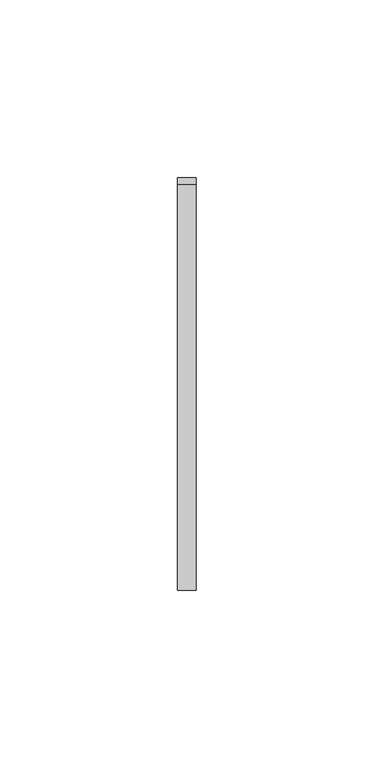
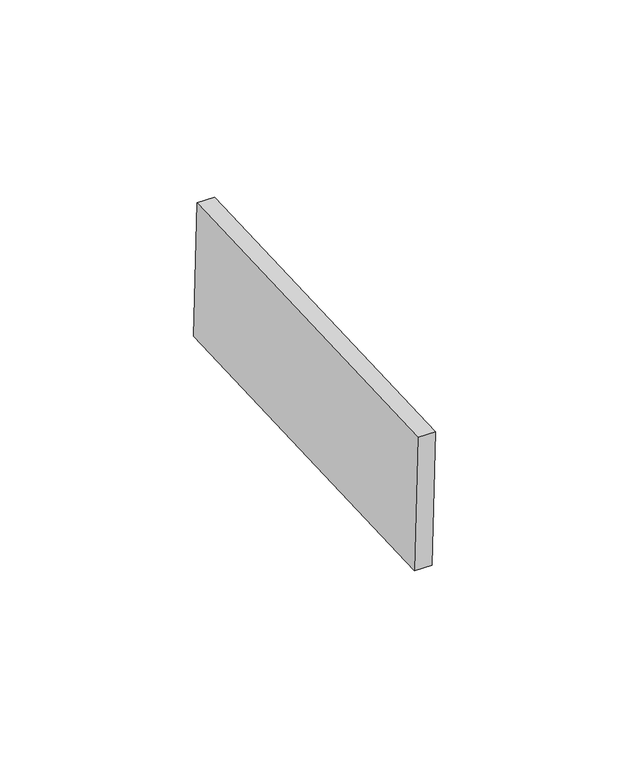
"""IFC4 building model written with IfcOpenShell, lengths in millimetres: proxy geometry, Inner panel:Inner panel:1:Inner panel:1 : Inner panel:Inner panel:300324:2:Inner panel:1:Inner panel:1 : Inner panel:Inner panel:300324:2 : Inner panel:Inner panel:1:Inner panel:1 : Inner panel:Inner panel:300324:300043:81 : Inner panel:Inner panel:1:Inner panel:1 : Inner panel:Inner panel:300324:2:Inner panel:1:Inner panel:1 : Inner panel:Inner panel:300324:2 : Inner panel:Inner panel:1:Inner panel:1 : Inner panel:Inner panel:300324:300043:308120."""

from ifc_helpers import new_model, si_unit, frame, origin, place, context, project, spatial, polyline, outline, extrude, source, transform, mapped, element, save


def generic_models_1863c1a6(model_context):
    return source(origin(), model_context, "Body", "SweptSolid", [
        extrude(outline(polyline([(0.0, -114.3), (0.0, 0.0), (5.2138089, 0.0), (5.2138089, -114.3), (0.0, -114.3)])), frame((592717.395117, -577458.3096573, 4016.6427799), z_axis=(0.0, -0.04163054471216399, 0.9991330730923527), x_axis=(-1.0, 0.0, 0.0)), (0.0, 0.0, 1.0), 43.2233908),
    ])


if __name__ == "__main__":
    model = new_model("IFC4")
    model_context = context("Model", 3, world=origin())
    ifc_project = project(units=[si_unit("LENGTHUNIT", "METRE", prefix="MILLI")], contexts=[model_context])
    site = spatial("IfcSite", under=ifc_project)
    building = spatial("IfcBuilding", under=site)
    placement = place(None, origin())
    generic_models_shape = generic_models_1863c1a6(model_context)
    element("IfcBuildingElementProxy", 1, Name="Inner panel:Inner panel:1:Inner panel:1 : Inner panel:Inner panel:300324:2:Inner panel:1:Inner panel:1 : Inner panel:Inner panel:300324:2 : Inner panel:Inner panel:1:Inner panel:1 : Inner panel:Inner panel:300324:300043:81 : Inner panel:Inner panel:1:Inner panel:1 : Inner panel:Inner panel:300324:2:Inner panel:1:Inner panel:1 : Inner panel:Inner panel:300324:2 : Inner panel:Inner panel:1:Inner panel:1 : Inner panel:Inner panel:300324:300043:308120", ObjectType="Inner panel:Inner panel:1:Inner panel:1 : Inner panel:Inner panel:300324:2:Inner panel:1:Inner panel:1 : Inner panel:Inner panel:300324:2 : Inner panel:Inner panel:1:Inner panel:1 : Inner panel:Inner panel:300324:300043:81 : Inner panel:Inner panel:1:Inner panel:1 : Inner panel:Inner panel:300324:2:Inner panel:1:Inner panel:1 : Inner panel:Inner panel:300324:2 : Inner panel:Inner panel:1:Inner panel:1 : Inner panel:Inner panel:300324:300043:308120", at=placement, inside=building, context=model_context, shape_type="MappedRepresentation", body=[
        mapped(generic_models_shape, transform((0.0, 0.0, 0.0), x_axis=(1.0, 0.0, 0.0), y_axis=(0.0, 1.0, 0.0), z_axis=(0.0, 0.0, 1.0))),
    ])
    save(model, "model.ifc")

# Revit data of these elements
# Type "Inner panel:Inner panel:1:Inner panel:1 : Inner panel:Inner panel:300324:2:Inner panel:1:Inner panel:1 : Inner panel:Inner panel:300324:2 : Inner panel:Inner panel:1:Inner panel:1 : Inner panel:Inner panel:300324:300043:81 : Inner panel:Inner panel:1:Inner panel:1 : Inner panel:Inner panel:300324:2:Inner panel:1:Inner panel:1 : Inner panel:Inner panel:300324:2 : Inner panel:Inner panel:1:Inner panel:1 : Inner panel:Inner panel:300324:300043:308120"
#   NameOverride = "Inner panel:Inner panel:1:Inner panel:1 : Inner panel:Inner panel:300324:2:Inner panel:1:Inner panel:1 : Inner panel:Inner panel:300324:2 : Inner panel:Inner panel:1:Inner panel:1 : Inner panel:Inner panel:300324:300043:308120"
#   ObjectTypeOverride = "Inner panel:1:Inner panel:1 : Inner panel:Inner panel:300324:2 : Inner panel:Inner panel:1:Inner panel:1 : Inner panel:Inner panel:300324:300043"
#   Reference = "Inner panel"
#   Tag = "308120"
# Element 1 (IfcBuildingElementProxy, "Inner panel:Inner panel:1:Inner panel:1 : Inner panel:Inner panel:300324:2:Inner panel:1:Inner panel:1 : Inner panel:Inner panel:300324:2 : Inner panel:Inner panel:1:Inner panel:1 : Inner panel:Inner panel:300324:300043:81 : Inner panel:Inner panel:1:Inner panel:1 : Inner panel:Inner panel:300324:2:Inner panel:1:Inner panel:1 : Inner panel:Inner panel:300324:2 : Inner panel:Inner panel:1:Inner panel:1 : Inner panel:Inner panel:300324:300043:308120")
#   Materials on its faces: "SLIDING CLIP"
# Materials
#   "SLIDING CLIP": class "Generic", colour RGB 120 120 120, transparency 0, Cost = 0
